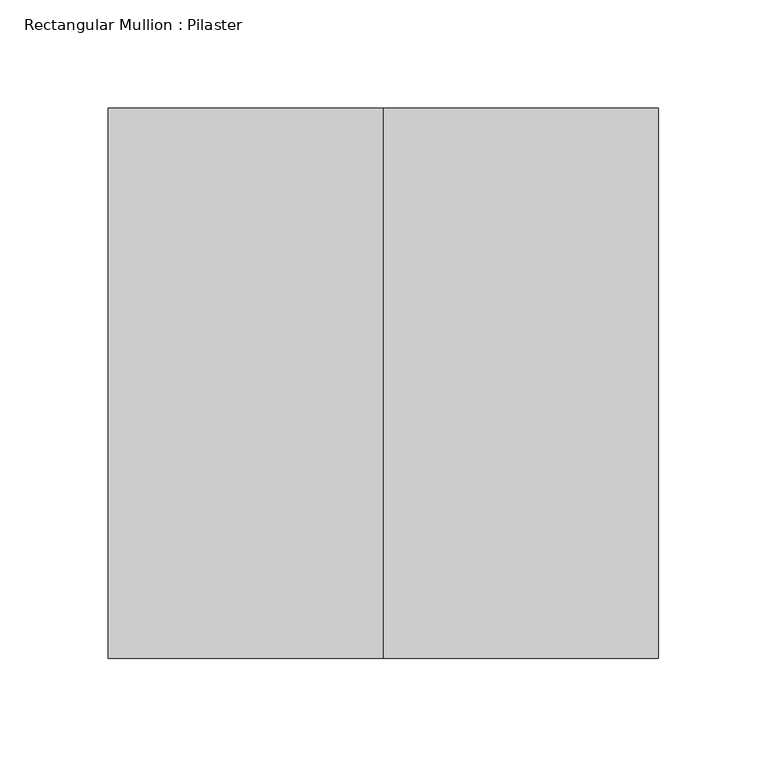
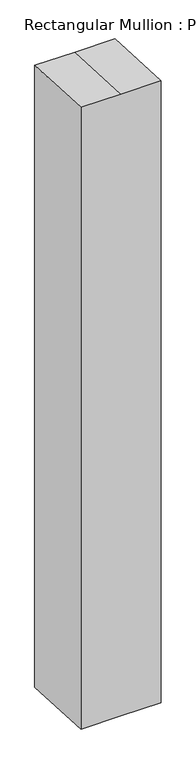
"""IFC4 building model written with IfcOpenShell, lengths in millimetres: member geometry, Rectangular Mullion : Pilaster."""

from ifc_helpers import new_model, si_unit, origin, place, context, project, spatial, faceted_brep, source, transform, mapped, element, save


def rectangular_mullion_pilaster_8c912226(model_context):
    return source(origin(), model_context, "Body", "Brep", [
        faceted_brep([(-127.0, 127.0, -7.074079), (0.0, 127.0, -7.074079), (127.0, 127.0, -7.074079), (127.0, 127.0, -2087.9711982), (0.0, 127.0, -2087.9711982), (-127.0, 127.0, -2087.9711982), (-127.0, -127.0, 6.2374969), (-127.0, -127.0, -2074.6596223), (127.0, -127.0, 6.2374969), (0.0, -127.0, 6.2374969), (0.0, -127.0, -2074.6596223), (127.0, -127.0, -2074.6596223)], [[[0, 1, 2, 3, 4, 5]], [[6, 0, 5, 7]], [[8, 9, 6, 7, 10, 11]], [[2, 8, 11, 3]], [[2, 1, 9, 8]], [[1, 0, 6, 9]], [[3, 11, 10, 4]], [[10, 7, 5, 4]]]),
    ])


if __name__ == "__main__":
    model = new_model("IFC4")
    model_context = context("Model", 3, world=origin())
    ifc_project = project(units=[si_unit("LENGTHUNIT", "METRE", prefix="MILLI")], contexts=[model_context])
    site = spatial("IfcSite", under=ifc_project)
    building = spatial("IfcBuilding", under=site)
    placement = place(None, origin())
    rectangular_mullion_pilaster_shape = rectangular_mullion_pilaster_8c912226(model_context)
    element("IfcMember", 1, ObjectType="Rectangular Mullion : Pilaster", at=placement, inside=building, context=model_context, shape_type="MappedRepresentation", body=[
        mapped(rectangular_mullion_pilaster_shape, transform((0.0, 0.0, 0.0), x_axis=(1.0, 0.0, 0.0), y_axis=(0.0, 1.0, 0.0), z_axis=(0.0, 0.0, 1.0))),
    ])
    save(model, "model.ifc")

# Revit data of these elements
# Type "Rectangular Mullion : Pilaster"
#   built-in parameter 1007304 = 0.833333 (stored number, unit not read)
#   built-in parameter 1007301 = 0.416667 (stored number, unit not read)
#   built-in parameter 1007300 = 0.416667 (stored number, unit not read)
# Element 1 (IfcMember, "Rectangular Mullion : Pilaster")
#   Materials on its faces: "Aluminum"
# Materials
#   "Aluminum": class "Metal", colour RGB 247 247 247, transparency 0, Description = "Aluminum 6061", Cost = 0
